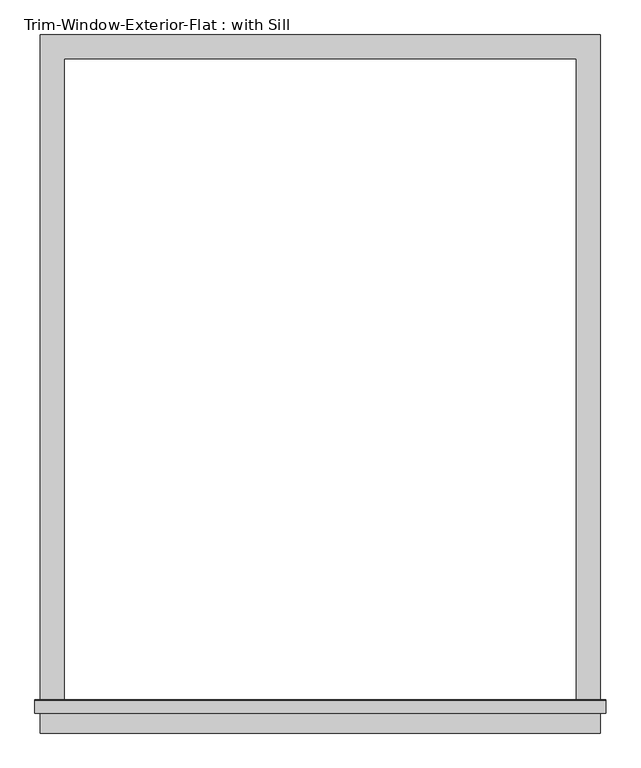
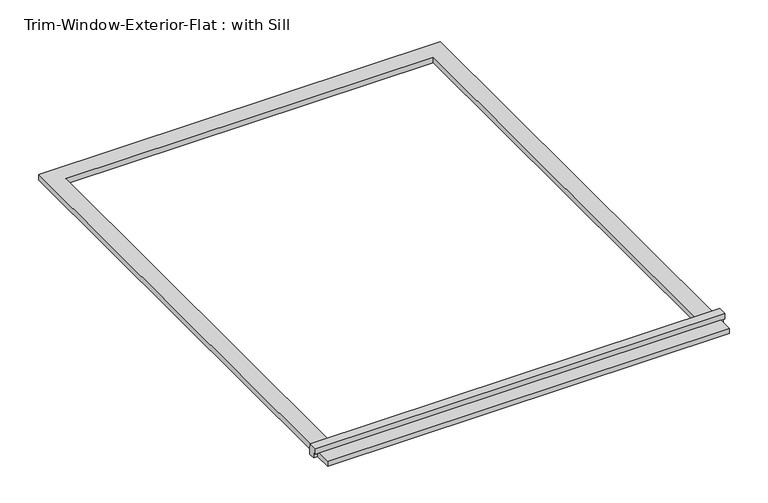
"""IFC4 building model written with IfcOpenShell, lengths in millimetres: proxy geometry, Trim-Window-Exterior-Flat : with Sill."""

import ifcopenshell
import ifcopenshell.guid

model = None  # the IFC model being written
_history = None  # IfcOwnerHistory: only IFC2X3 demands one
_inside = {}  # id of a spatial element -> (the spatial element, [elements in it])
_under = {}  # id of a project, library or spatial element -> (it, [spatial elements below it])
_declared = {}  # id of a project -> (the project, [libraries it declares])
_typed = {}  # id of a type object -> (the type object, [elements of that type])
_made_of = {}  # id of a material, layer set ... -> (it, [elements and type objects made of it])


def new_model(schema):
    """Start an empty IFC model of exactly this schema.

    Asked for "IFC4X3", IfcOpenShell would pick the latest addendum, in which some entities
    have other attributes; the version numbers below select the first issue.
    IFC2X3 requires an IfcOwnerHistory on every rooted entity: one is made here for all.
    """
    global model, _history
    if schema == "IFC4X3":
        model = ifcopenshell.file(schema_version=(4, 3, 0, 0))
    else:
        model = ifcopenshell.file(schema=schema)
    _inside.clear()
    _under.clear()
    _declared.clear()
    _typed.clear()
    _made_of.clear()
    _history = None
    if model.schema == "IFC2X3":
        org = make("IfcOrganization", Name="unknown")
        user = make(
            "IfcPersonAndOrganization",
            ThePerson=make("IfcPerson", FamilyName="unknown"),
            TheOrganization=org,
        )
        app = make(
            "IfcApplication",
            ApplicationDeveloper=org,
            Version="unknown",
            ApplicationFullName="unknown",
            ApplicationIdentifier="unknown",
        )
        _history = make(
            "IfcOwnerHistory",
            OwningUser=user,
            OwningApplication=app,
            ChangeAction="ADDED",
            CreationDate=0,
        )
    return model


def make(cls, **values):
    """One entity of the class cls with the attributes given. An attribute that is None is left unset."""
    return model.create_entity(
        cls, **{name: value for name, value in values.items() if value is not None}
    )


def rooted(cls, **values):
    """An entity with a GlobalId (a new one), such as an element, a storey or a relation."""
    return make(cls, GlobalId=ifcopenshell.guid.new(), OwnerHistory=_history, **values)


def si_unit(unit_type, name, prefix=None):
    """IfcSIUnit, for example si_unit("LENGTHUNIT", "METRE", prefix="MILLI")."""
    return make("IfcSIUnit", UnitType=unit_type, Prefix=prefix, Name=name)


def assignment(units):
    """IfcUnitAssignment: the units of a project."""
    return None if units is None else make("IfcUnitAssignment", Units=units)


def point(xyz):
    """IfcCartesianPoint."""
    return None if xyz is None else make("IfcCartesianPoint", Coordinates=xyz)


def direction(xyz):
    """IfcDirection."""
    return None if xyz is None else make("IfcDirection", DirectionRatios=xyz)


def frame(location, z_axis=None, x_axis=None):
    """IfcAxis2Placement3D, a coordinate frame: its origin and axes. An axis left out is left unset."""
    return make(
        "IfcAxis2Placement3D",
        Location=point(location),
        Axis=direction(z_axis),
        RefDirection=direction(x_axis),
    )


def origin():
    """The frame at (0, 0, 0) with its axes left unset."""
    return frame((0.0, 0.0, 0.0))


def origin_with_axes():
    """The frame at (0, 0, 0) with the z axis (0, 0, 1) and the x axis (1, 0, 0) written out."""
    return frame((0.0, 0.0, 0.0), z_axis=(0.0, 0.0, 1.0), x_axis=(1.0, 0.0, 0.0))


def place(relative_to, where):
    """IfcLocalPlacement: puts the frame where relative to a parent placement (None: the world)."""
    return make(
        "IfcLocalPlacement", PlacementRelTo=relative_to, RelativePlacement=where
    )


def context(
    kind, dimensions, precision=None, world=None, true_north=None, identifier=None
):
    """IfcGeometricRepresentationContext, for example the 3D "Model" context."""
    return make(
        "IfcGeometricRepresentationContext",
        ContextIdentifier=identifier,
        ContextType=kind,
        CoordinateSpaceDimension=dimensions,
        Precision=precision,
        WorldCoordinateSystem=world,
        TrueNorth=true_north,
    )


def project(units=None, contexts=None):
    """IfcProject with its units and contexts."""
    return rooted(
        "IfcProject",
        Name="project",
        RepresentationContexts=contexts,
        UnitsInContext=assignment(units),
    )


def spatial(cls, under=None, at=None, **own):
    """A site, building, storey or space (cls), placed at a placement, below another one or the project."""
    s = rooted(cls, ObjectPlacement=at, **own)
    if under is not None:
        _under.setdefault(under.id(), (under, []))[1].append(s)
    return s


def polyline(points):
    """IfcPolyline through the points."""
    return make("IfcPolyline", Points=[point(p) for p in points])


def outline(outer, holes=None, kind="AREA"):
    """IfcArbitraryClosedProfileDef: a profile drawn as a closed curve; with holes, ...WithVoids."""
    if holes is None:
        return make("IfcArbitraryClosedProfileDef", ProfileType=kind, OuterCurve=outer)
    return make(
        "IfcArbitraryProfileDefWithVoids",
        ProfileType=kind,
        OuterCurve=outer,
        InnerCurves=holes,
    )


def extrude(swept, where, along, depth):
    """IfcExtrudedAreaSolid: the profile swept, set in the frame where, extruded along a direction by depth."""
    return make(
        "IfcExtrudedAreaSolid",
        SweptArea=swept,
        Position=where,
        ExtrudedDirection=direction(along),
        Depth=depth,
    )


def shape(context_of_items, identifier, shape_type, items):
    """IfcShapeRepresentation: the items that make up one representation, for example the "Body"."""
    return make(
        "IfcShapeRepresentation",
        ContextOfItems=context_of_items,
        RepresentationIdentifier=identifier,
        RepresentationType=shape_type,
        Items=items,
    )


def source(mapping_origin, context_of_items, identifier, shape_type, items):
    """IfcRepresentationMap: a shape defined once, which mapped items show again and again."""
    return make(
        "IfcRepresentationMap",
        MappingOrigin=mapping_origin,
        MappedRepresentation=shape(context_of_items, identifier, shape_type, items),
    )


def transform(
    local_origin,
    x_axis=None,
    y_axis=None,
    z_axis=None,
    scale=None,
    scale2=None,
    scale3=None,
    uniform=True,
):
    """IfcCartesianTransformationOperator3D, or its non-uniform kind. x_axis, y_axis, z_axis: its Axis1, 2, 3."""
    if uniform:
        return make(
            "IfcCartesianTransformationOperator3D",
            Axis1=direction(x_axis),
            Axis2=direction(y_axis),
            LocalOrigin=point(local_origin),
            Scale=scale,
            Axis3=direction(z_axis),
        )
    return make(
        "IfcCartesianTransformationOperator3DnonUniform",
        Axis1=direction(x_axis),
        Axis2=direction(y_axis),
        LocalOrigin=point(local_origin),
        Scale=scale,
        Axis3=direction(z_axis),
        Scale2=scale2,
        Scale3=scale3,
    )


def mapped(mapping_source, mapping_target):
    """IfcMappedItem: shows the shape of a source again, moved by a transform."""
    return make(
        "IfcMappedItem", MappingSource=mapping_source, MappingTarget=mapping_target
    )


def made_of(thing, what):
    """Note that an element or type object is made of a material, layer set ...; save() writes the relation."""
    if what is not None:
        _made_of.setdefault(what.id(), (what, []))[1].append(thing)
    return thing


def element(
    cls,
    number,
    at=None,
    inside=None,
    cuts=None,
    type_object=None,
    material=None,
    context=None,
    identifier="Body",
    shape_type=None,
    held_by="IfcProductDefinitionShape",
    body=None,
    shapes=None,
    **own,
):
    """One element of the class cls, such as IfcWall. Its Tag is "e" and its number.

    at: its placement. inside: the storey or other place that contains it. cuts: it is an
    opening in that element (IfcRelVoidsElement). A single representation is given by context,
    identifier, shape_type and body (its items); several are given by shapes. held_by: the class
    of the entity that holds the representations. save() writes the other relations.
    """
    e = rooted(cls, Tag="e%d" % number, ObjectPlacement=at, **own)
    if body is not None:
        shapes = [shape(context, identifier, shape_type, body)]
    if shapes is not None:
        e.Representation = make(held_by, Representations=shapes)
    if inside is not None:
        _inside.setdefault(inside.id(), (inside, []))[1].append(e)
    if cuts is not None:
        rooted(
            "IfcRelVoidsElement", RelatingBuildingElement=cuts, RelatedOpeningElement=e
        )
    if type_object is not None:
        _typed.setdefault(type_object.id(), (type_object, []))[1].append(e)
    return made_of(e, material)


def aggregate(whole, parts):
    """IfcRelAggregates: a whole, such as a stair, and the parts it consists of."""
    return rooted("IfcRelAggregates", RelatingObject=whole, RelatedObjects=parts)


def save(model, path):
    """Write the relations noted so far, then the file.

    IfcRelAggregates (storeys below a building ...), IfcRelContainedInSpatialStructure (elements
    in a storey), IfcRelDefinesByType, IfcRelAssociatesMaterial and IfcRelDeclares: one each for
    every whole, place, type object, material and project.
    """
    for whole, parts in _under.values():
        aggregate(whole, parts)
    for where, things in _inside.values():
        rooted(
            "IfcRelContainedInSpatialStructure",
            RelatedElements=things,
            RelatingStructure=where,
        )
    for kind, things in _typed.values():
        rooted("IfcRelDefinesByType", RelatedObjects=things, RelatingType=kind)
    for what, things in _made_of.values():
        rooted("IfcRelAssociatesMaterial", RelatedObjects=things, RelatingMaterial=what)
    for by, libraries in _declared.values():
        rooted("IfcRelDeclares", RelatingContext=by, RelatedDefinitions=libraries)
    model.write(path)


def trim_window_exterior_flat_with_sill_92b9b949(model_context):
    return source(origin(), model_context, "Body", "SweptSolid", [
        extrude(outline(polyline([(666.75, -1546.1823709), (666.75, -1603.3323709), (-666.75, -1603.3323709), (-666.75, -1546.1823709), (666.75, -1546.1823709)])), origin_with_axes(), (0.0, 0.0, 1.0), 19.05),
        extrude(outline(polyline([(-1555.75, 38.1), (-1526.4580645, 38.1), (-1524.0, 19.05), (-1524.0, 0.0), (-1546.1823709, 0.0), (-1546.1823709, 19.05), (-1555.75, 19.05), (-1555.75, 38.1)])), frame((-679.45, 0.0, 0.0), z_axis=(1.0, 0.0, 0.0), x_axis=(0.0, 1.0, 0.0)), (0.0, 0.0, 1.0), 1358.9),
        extrude(outline(polyline([(-666.75, 57.15), (666.75, 57.15), (666.75, -1524.0), (609.6, -1524.0), (609.6, 0.0), (-609.6, 0.0), (-609.6, -1524.0), (-666.75, -1524.0), (-666.75, 57.15)])), origin_with_axes(), (0.0, 0.0, 1.0), 19.05),
    ])


if __name__ == "__main__":
    model = new_model("IFC4")
    model_context = context("Model", 3, world=origin())
    ifc_project = project(units=[si_unit("LENGTHUNIT", "METRE", prefix="MILLI")], contexts=[model_context])
    site = spatial("IfcSite", under=ifc_project)
    building = spatial("IfcBuilding", under=site)
    placement = place(None, origin())
    trim_window_exterior_flat_with_sill_shape = trim_window_exterior_flat_with_sill_92b9b949(model_context)
    element("IfcBuildingElementProxy", 1, Name="Trim-Window-Exterior-Flat : with Sill", ObjectType="Trim-Window-Exterior-Flat : with Sill", at=placement, inside=building, context=model_context, shape_type="MappedRepresentation", body=[
        mapped(trim_window_exterior_flat_with_sill_shape, transform((0.0, 0.0, 0.0), x_axis=(1.0, 0.0, 0.0), y_axis=(0.0, 1.0, 0.0), z_axis=(0.0, 0.0, 1.0))),
    ])
    save(model, "model.ifc")

# Revit data of these elements
# Type "Trim-Window-Exterior-Flat : with Sill"
#   Trim Width = 0' - 2 1/4"
#   Trim Thickness_Picture Frame = 0' - 1 1/4"
#   Trim Thickness_with Sill = 0' - 0 3/4"
#   Sill Thickness = 0' - 1 1/4"
#   Opening Width [instance default] = 2' - 0"
#   Opening Height [instance default] = 3' - 0"
#   Default Elevation = 4' - 0"
#   Sill = yes
#   Picture Frame = no
#   Trim Material [instance default] = none
# Element 1 (IfcBuildingElementProxy, "Trim-Window-Exterior-Flat : with Sill")
#   Opening Width = 4' - 0"
#   Opening Height = 5' - 0"
#   Trim Material = Clad - White
#   Materials on its faces: "Clad - White"
# Materials
#   "Clad - White": class "Wood", colour RGB 216 216 204, transparency 0, Cost = 0
